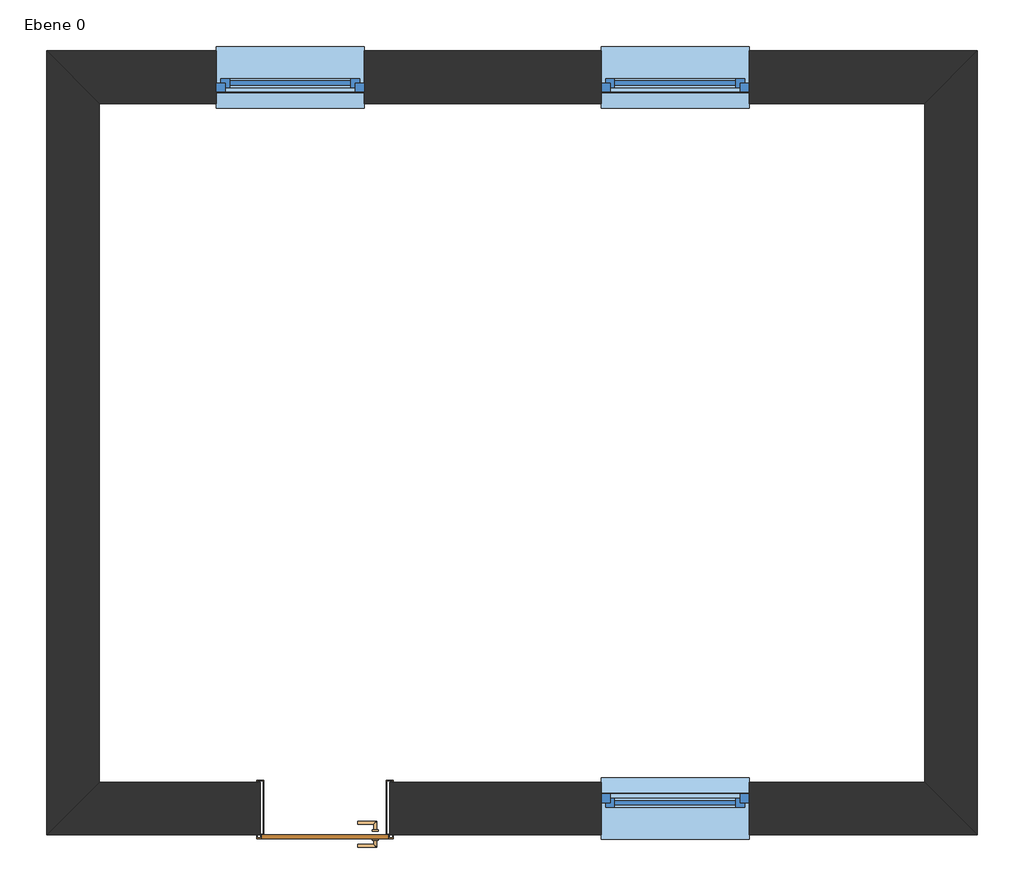
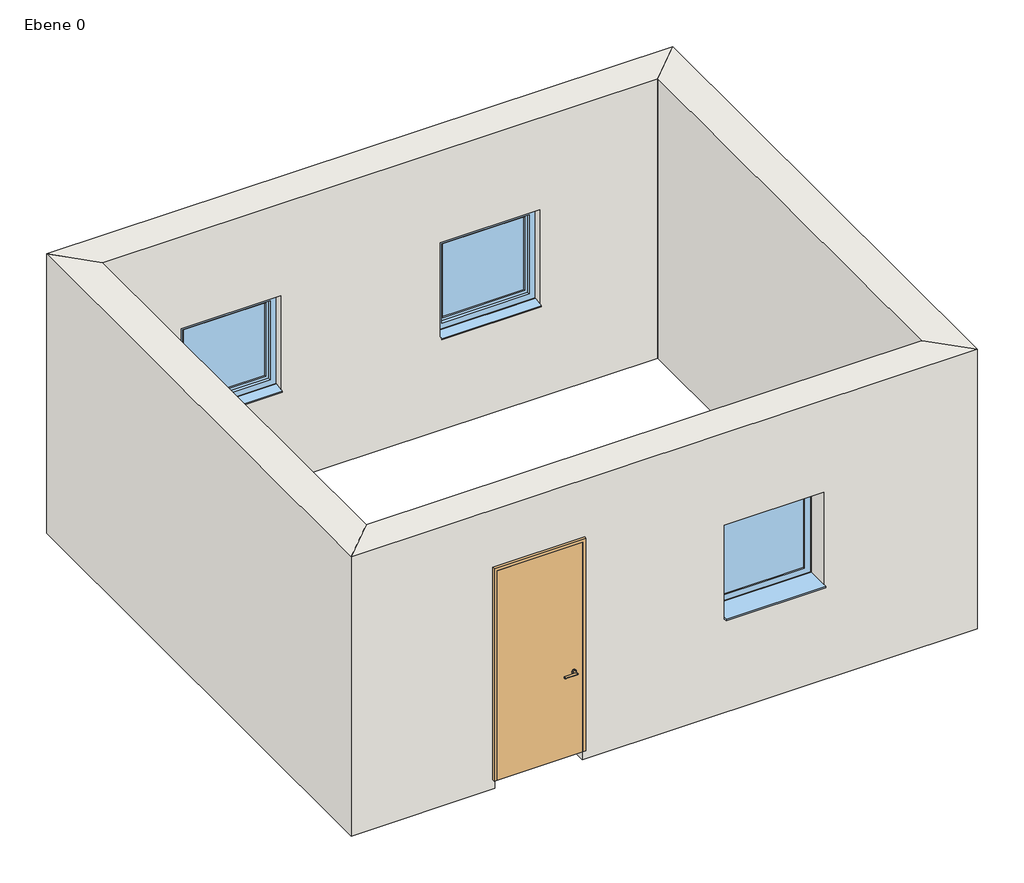
# One storey: 4 walls, 3 windows, 1 door.
"""IFC4 building model written with IfcOpenShell, lengths in millimetres."""

import ifcopenshell
import ifcopenshell.guid

model = None  # the IFC model being written
_history = None  # IfcOwnerHistory: only IFC2X3 demands one
_inside = {}  # id of a spatial element -> (the spatial element, [elements in it])
_under = {}  # id of a project, library or spatial element -> (it, [spatial elements below it])
_declared = {}  # id of a project -> (the project, [libraries it declares])
_typed = {}  # id of a type object -> (the type object, [elements of that type])
_made_of = {}  # id of a material, layer set ... -> (it, [elements and type objects made of it])


def new_model(schema):
    """Start an empty IFC model of exactly this schema.

    Asked for "IFC4X3", IfcOpenShell would pick the latest addendum, in which some entities
    have other attributes; the version numbers below select the first issue.
    IFC2X3 requires an IfcOwnerHistory on every rooted entity: one is made here for all.
    """
    global model, _history
    if schema == "IFC4X3":
        model = ifcopenshell.file(schema_version=(4, 3, 0, 0))
    else:
        model = ifcopenshell.file(schema=schema)
    _inside.clear()
    _under.clear()
    _declared.clear()
    _typed.clear()
    _made_of.clear()
    _history = None
    if model.schema == "IFC2X3":
        org = make("IfcOrganization", Name="unknown")
        user = make(
            "IfcPersonAndOrganization",
            ThePerson=make("IfcPerson", FamilyName="unknown"),
            TheOrganization=org,
        )
        app = make(
            "IfcApplication",
            ApplicationDeveloper=org,
            Version="unknown",
            ApplicationFullName="unknown",
            ApplicationIdentifier="unknown",
        )
        _history = make(
            "IfcOwnerHistory",
            OwningUser=user,
            OwningApplication=app,
            ChangeAction="ADDED",
            CreationDate=0,
        )
    return model


def make(cls, **values):
    """One entity of the class cls with the attributes given. An attribute that is None is left unset."""
    return model.create_entity(
        cls, **{name: value for name, value in values.items() if value is not None}
    )


def rooted(cls, **values):
    """An entity with a GlobalId (a new one), such as an element, a storey or a relation."""
    return make(cls, GlobalId=ifcopenshell.guid.new(), OwnerHistory=_history, **values)


def si_unit(unit_type, name, prefix=None):
    """IfcSIUnit, for example si_unit("LENGTHUNIT", "METRE", prefix="MILLI")."""
    return make("IfcSIUnit", UnitType=unit_type, Prefix=prefix, Name=name)


def assignment(units):
    """IfcUnitAssignment: the units of a project."""
    return None if units is None else make("IfcUnitAssignment", Units=units)


def point(xyz):
    """IfcCartesianPoint."""
    return None if xyz is None else make("IfcCartesianPoint", Coordinates=xyz)


def direction(xyz):
    """IfcDirection."""
    return None if xyz is None else make("IfcDirection", DirectionRatios=xyz)


def frame(location, z_axis=None, x_axis=None):
    """IfcAxis2Placement3D, a coordinate frame: its origin and axes. An axis left out is left unset."""
    return make(
        "IfcAxis2Placement3D",
        Location=point(location),
        Axis=direction(z_axis),
        RefDirection=direction(x_axis),
    )


def frame_2d(location, x_axis=None):
    """IfcAxis2Placement2D, a coordinate frame in the plane: its origin and x axis."""
    return make(
        "IfcAxis2Placement2D", Location=point(location), RefDirection=direction(x_axis)
    )


def origin():
    """The frame at (0, 0, 0) with its axes left unset."""
    return frame((0.0, 0.0, 0.0))


def origin_with_axes():
    """The frame at (0, 0, 0) with the z axis (0, 0, 1) and the x axis (1, 0, 0) written out."""
    return frame((0.0, 0.0, 0.0), z_axis=(0.0, 0.0, 1.0), x_axis=(1.0, 0.0, 0.0))


def place(relative_to, where):
    """IfcLocalPlacement: puts the frame where relative to a parent placement (None: the world)."""
    return make(
        "IfcLocalPlacement", PlacementRelTo=relative_to, RelativePlacement=where
    )


def context(
    kind, dimensions, precision=None, world=None, true_north=None, identifier=None
):
    """IfcGeometricRepresentationContext, for example the 3D "Model" context."""
    return make(
        "IfcGeometricRepresentationContext",
        ContextIdentifier=identifier,
        ContextType=kind,
        CoordinateSpaceDimension=dimensions,
        Precision=precision,
        WorldCoordinateSystem=world,
        TrueNorth=true_north,
    )


def project(units=None, contexts=None):
    """IfcProject with its units and contexts."""
    return rooted(
        "IfcProject",
        Name="project",
        RepresentationContexts=contexts,
        UnitsInContext=assignment(units),
    )


def spatial(cls, under=None, at=None, **own):
    """A site, building, storey or space (cls), placed at a placement, below another one or the project."""
    s = rooted(cls, ObjectPlacement=at, **own)
    if under is not None:
        _under.setdefault(under.id(), (under, []))[1].append(s)
    return s


def polyline(points):
    """IfcPolyline through the points."""
    return make("IfcPolyline", Points=[point(p) for p in points])


def circle_curve(where, radius):
    """IfcCircle in the frame where."""
    return make("IfcCircle", Position=where, Radius=radius)


def ellipse_curve(where, semi_axis1, semi_axis2):
    """IfcEllipse in the frame where."""
    return make(
        "IfcEllipse", Position=where, SemiAxis1=semi_axis1, SemiAxis2=semi_axis2
    )


def trimmed(basis, trim1, trim2, sense, master):
    """IfcTrimmedCurve: the piece of a basis curve between two trims."""
    return make(
        "IfcTrimmedCurve",
        BasisCurve=basis,
        Trim1=trim1,
        Trim2=trim2,
        SenseAgreement=sense,
        MasterRepresentation=master,
    )


def segment(curve, same_sense, transition):
    """IfcCompositeCurveSegment."""
    return make(
        "IfcCompositeCurveSegment",
        Transition=transition,
        SameSense=same_sense,
        ParentCurve=curve,
    )


def composite_curve(segments, self_intersect=None):
    """IfcCompositeCurve: segments joined end to end."""
    return make("IfcCompositeCurve", Segments=segments, SelfIntersect=self_intersect)


def outline(outer, holes=None, kind="AREA"):
    """IfcArbitraryClosedProfileDef: a profile drawn as a closed curve; with holes, ...WithVoids."""
    if holes is None:
        return make("IfcArbitraryClosedProfileDef", ProfileType=kind, OuterCurve=outer)
    return make(
        "IfcArbitraryProfileDefWithVoids",
        ProfileType=kind,
        OuterCurve=outer,
        InnerCurves=holes,
    )


def extrude(swept, where, along, depth):
    """IfcExtrudedAreaSolid: the profile swept, set in the frame where, extruded along a direction by depth."""
    return make(
        "IfcExtrudedAreaSolid",
        SweptArea=swept,
        Position=where,
        ExtrudedDirection=direction(along),
        Depth=depth,
    )


def faces_of(points, faces, orient=None, outer=None):
    """IfcFace entities. A face is a list of loops; a loop is a list of indices into points, from 0.

    orient and outer hold one flag for each loop. By default every Orientation is true, the
    first loop of a face is its IfcFaceOuterBound and the others are IfcFaceBound.
    """
    made = []
    for i, loops in enumerate(faces):
        bounds = []
        for j, loop in enumerate(loops):
            is_outer = j == 0 if outer is None else outer[i][j]
            bounds.append(
                make(
                    "IfcFaceOuterBound" if is_outer else "IfcFaceBound",
                    Bound=make("IfcPolyLoop", Polygon=[points[k] for k in loop]),
                    Orientation=True if orient is None else orient[i][j],
                )
            )
        made.append(make("IfcFace", Bounds=bounds))
    return made


def faceted_brep(points, faces, orient=None, outer=None, voids=None):
    """IfcFacetedBrep: a solid bounded by flat faces; with voids (closed shells), ...WithVoids."""
    shared = [point(p) for p in points]
    hull = make("IfcClosedShell", CfsFaces=faces_of(shared, faces, orient, outer))
    if voids is None:
        return make("IfcFacetedBrep", Outer=hull)
    return make(
        "IfcFacetedBrepWithVoids",
        Outer=hull,
        Voids=[
            make(cls, CfsFaces=faces_of(shared, fs, o, b)) for cls, fs, o, b in voids
        ],
    )


def shape(context_of_items, identifier, shape_type, items):
    """IfcShapeRepresentation: the items that make up one representation, for example the "Body"."""
    return make(
        "IfcShapeRepresentation",
        ContextOfItems=context_of_items,
        RepresentationIdentifier=identifier,
        RepresentationType=shape_type,
        Items=items,
    )


def source(mapping_origin, context_of_items, identifier, shape_type, items):
    """IfcRepresentationMap: a shape defined once, which mapped items show again and again."""
    return make(
        "IfcRepresentationMap",
        MappingOrigin=mapping_origin,
        MappedRepresentation=shape(context_of_items, identifier, shape_type, items),
    )


def transform(
    local_origin,
    x_axis=None,
    y_axis=None,
    z_axis=None,
    scale=None,
    scale2=None,
    scale3=None,
    uniform=True,
):
    """IfcCartesianTransformationOperator3D, or its non-uniform kind. x_axis, y_axis, z_axis: its Axis1, 2, 3."""
    if uniform:
        return make(
            "IfcCartesianTransformationOperator3D",
            Axis1=direction(x_axis),
            Axis2=direction(y_axis),
            LocalOrigin=point(local_origin),
            Scale=scale,
            Axis3=direction(z_axis),
        )
    return make(
        "IfcCartesianTransformationOperator3DnonUniform",
        Axis1=direction(x_axis),
        Axis2=direction(y_axis),
        LocalOrigin=point(local_origin),
        Scale=scale,
        Axis3=direction(z_axis),
        Scale2=scale2,
        Scale3=scale3,
    )


def mapped(mapping_source, mapping_target):
    """IfcMappedItem: shows the shape of a source again, moved by a transform."""
    return make(
        "IfcMappedItem", MappingSource=mapping_source, MappingTarget=mapping_target
    )


def made_of(thing, what):
    """Note that an element or type object is made of a material, layer set ...; save() writes the relation."""
    if what is not None:
        _made_of.setdefault(what.id(), (what, []))[1].append(thing)
    return thing


def element(
    cls,
    number,
    at=None,
    inside=None,
    cuts=None,
    type_object=None,
    material=None,
    context=None,
    identifier="Body",
    shape_type=None,
    held_by="IfcProductDefinitionShape",
    body=None,
    shapes=None,
    **own,
):
    """One element of the class cls, such as IfcWall. Its Tag is "e" and its number.

    at: its placement. inside: the storey or other place that contains it. cuts: it is an
    opening in that element (IfcRelVoidsElement). A single representation is given by context,
    identifier, shape_type and body (its items); several are given by shapes. held_by: the class
    of the entity that holds the representations. save() writes the other relations.
    """
    e = rooted(cls, Tag="e%d" % number, ObjectPlacement=at, **own)
    if body is not None:
        shapes = [shape(context, identifier, shape_type, body)]
    if shapes is not None:
        e.Representation = make(held_by, Representations=shapes)
    if inside is not None:
        _inside.setdefault(inside.id(), (inside, []))[1].append(e)
    if cuts is not None:
        rooted(
            "IfcRelVoidsElement", RelatingBuildingElement=cuts, RelatedOpeningElement=e
        )
    if type_object is not None:
        _typed.setdefault(type_object.id(), (type_object, []))[1].append(e)
    return made_of(e, material)


def aggregate(whole, parts):
    """IfcRelAggregates: a whole, such as a stair, and the parts it consists of."""
    return rooted("IfcRelAggregates", RelatingObject=whole, RelatedObjects=parts)


def save(model, path):
    """Write the relations noted so far, then the file.

    IfcRelAggregates (storeys below a building ...), IfcRelContainedInSpatialStructure (elements
    in a storey), IfcRelDefinesByType, IfcRelAssociatesMaterial and IfcRelDeclares: one each for
    every whole, place, type object, material and project.
    """
    for whole, parts in _under.values():
        aggregate(whole, parts)
    for where, things in _inside.values():
        rooted(
            "IfcRelContainedInSpatialStructure",
            RelatedElements=things,
            RelatingStructure=where,
        )
    for kind, things in _typed.values():
        rooted("IfcRelDefinesByType", RelatedObjects=things, RelatingType=kind)
    for what, things in _made_of.values():
        rooted("IfcRelAssociatesMaterial", RelatedObjects=things, RelatingMaterial=what)
    for by, libraries in _declared.values():
        rooted("IfcRelDeclares", RelatingContext=by, RelatedDefinitions=libraries)
    model.write(path)


def plane_surface(at):
    """IfcPlane: the flat surface through the origin of the frame at, square to its z axis."""
    return make("IfcPlane", Position=at)


def cylinder_surface(at, radius):
    """IfcCylindricalSurface: all points at the distance radius from the z axis of the frame at."""
    return make("IfcCylindricalSurface", Position=at, Radius=radius)


def advanced_brep(points, edges, surfaces, faces):
    """IfcAdvancedBrep: a solid bounded by faces that lie on surfaces and meet in shared edges.

    An edge is (start, end): straight between two places in points (the first is 0);
    or (start, end, curve); or (start, end, curve, False) where it runs against its curve.
    A face is (place in surfaces, loops), or (place, loops, False) where it looks against
    its surface's normal. A loop lists edges by number (the first is 1), with a minus sign
    where the edge is run from its end to its start. The first loop is the outer one.
    """
    corners = [point(p) for p in points]
    vertices = [make("IfcVertexPoint", VertexGeometry=c) for c in corners]
    made = []
    for start, end, *more in edges:
        made.append(
            make(
                "IfcEdgeCurve",
                EdgeStart=vertices[start],
                EdgeEnd=vertices[end],
                EdgeGeometry=more[0] if more else make("IfcPolyline", Points=[corners[start], corners[end]]),
                SameSense=more[1] if len(more) > 1 else True,
            )
        )
    hull = []
    for where, loops, *sense in faces:
        bounds = []
        for j, loop in enumerate(loops):
            ring = [make("IfcOrientedEdge", EdgeElement=made[abs(k) - 1], Orientation=k > 0) for k in loop]
            bounds.append(
                make(
                    "IfcFaceOuterBound" if j == 0 else "IfcFaceBound",
                    Bound=make("IfcEdgeLoop", EdgeList=ring),
                    Orientation=True,
                )
            )
        hull.append(make("IfcAdvancedFace", Bounds=bounds, FaceSurface=surfaces[where], SameSense=sense[0] if sense else True))
    return make("IfcAdvancedBrep", Outer=make("IfcClosedShell", CfsFaces=hull))


def door_88_5_x_2_26_80f06d6c(model_context):
    return source(origin(), model_context, "Body", "SolidModel", [
        advanced_brep(
        [(-352.5, 169.4346141, 1000.0), (-332.5, 169.4346141, 1000.0), (-352.5, 99.4346141, 1000.0), (-332.5, 119.4346141, 1000.0), (-222.5, 99.4346141, 1000.0), (-222.5, 119.4346141, 1000.0)],
        [
            (0, 1, circle_curve(frame((-342.5, 169.4346141, 1000.0), z_axis=(0.0, 1.0, 0.0), x_axis=(1.0, 0.0, 0.0)), 10.0)),
            (1, 0, circle_curve(frame((-342.5, 169.4346141, 1000.0), z_axis=(0.0, 1.0, 0.0), x_axis=(1.0, 0.0, 0.0)), 10.0)),
            (0, 2),
            (2, 3, ellipse_curve(frame((-342.5, 109.4346141, 1000.0), z_axis=(-0.7071067811865385, 0.7071067811865565, 0.0), x_axis=(0.7071067811865563, 0.7071067811865386, 0.0)), 14.1421356, 10.0)),
            (3, 1),
            (3, 2, ellipse_curve(frame((-342.5, 109.4346141, 1000.0), z_axis=(-0.7071067811865385, 0.7071067811865565, 0.0), x_axis=(0.7071067811865563, 0.7071067811865386, 0.0)), 14.1421356, 10.0)),
            (4, 5, circle_curve(frame((-222.5, 109.4346141, 1000.0), z_axis=(1.0, 0.0, 0.0), x_axis=(0.0, 1.0, 0.0)), 10.0)),
            (5, 4, circle_curve(frame((-222.5, 109.4346141, 1000.0), z_axis=(1.0, 0.0, 0.0), x_axis=(0.0, 1.0, 0.0)), 10.0)),
            (2, 4),
            (5, 3),
        ],
        [
            plane_surface(frame((-342.5, 169.4346141, -287.7526403), z_axis=(0.0, 1.0, 0.0), x_axis=(0.0, 0.0, 1.0))),
            cylinder_surface(frame((-342.5, 169.4346141, 1000.0), z_axis=(0.0, 1.0, 0.0), x_axis=(1.0, 0.0, 0.0)), 10.0),
            plane_surface(frame((-222.5, 109.4346141, -287.7526403), z_axis=(1.0, 0.0, 0.0), x_axis=(0.0, 0.0, 1.0))),
            cylinder_surface(frame((-342.5, 109.4346141, 1000.0), z_axis=(-1.0, 0.0, 0.0), x_axis=(0.0, 1.0, 0.0)), 10.0),
        ],
        [
            (0, [[1, 2]]),
            (1, [[-1, 3, 4, 5]]),
            (1, [[-2, -5, 6, -3]]),
            (2, [[7, 8]]),
            (3, [[-4, 9, -8, 10]]),
            (3, [[-6, -10, -7, -9]]),
        ],
    ),
        advanced_brep(
        [(-332.5, 229.4346141, 1000.0), (-352.5, 229.4346141, 1000.0), (-332.5, 259.4346141, 1000.0), (-352.5, 279.4346141, 1000.0), (-222.5, 259.4346141, 1000.0), (-222.5, 279.4346141, 1000.0)],
        [
            (0, 1, circle_curve(frame((-342.5, 229.4346141, 1000.0), z_axis=(0.0, -1.0, 0.0), x_axis=(-1.0, 0.0, 0.0)), 10.0)),
            (1, 0, circle_curve(frame((-342.5, 229.4346141, 1000.0), z_axis=(0.0, -1.0, 0.0), x_axis=(-1.0, 0.0, 0.0)), 10.0)),
            (0, 2),
            (2, 3, ellipse_curve(frame((-342.5, 269.4346141, 1000.0), z_axis=(-0.7071067811865475, -0.7071067811865475, 0.0), x_axis=(0.7071067811865474, -0.7071067811865476, 0.0)), 14.1421356, 10.0)),
            (3, 1),
            (3, 2, ellipse_curve(frame((-342.5, 269.4346141, 1000.0), z_axis=(-0.7071067811865475, -0.7071067811865475, 0.0), x_axis=(0.7071067811865474, -0.7071067811865476, 0.0)), 14.1421356, 10.0)),
            (4, 5, circle_curve(frame((-222.5, 269.4346141, 1000.0), z_axis=(1.0, 0.0, 0.0), x_axis=(0.0, 1.0, 0.0)), 10.0)),
            (5, 4, circle_curve(frame((-222.5, 269.4346141, 1000.0), z_axis=(1.0, 0.0, 0.0), x_axis=(0.0, 1.0, 0.0)), 10.0)),
            (2, 4),
            (5, 3),
        ],
        [
            plane_surface(frame((-342.5, 229.4346141, -287.7526403), z_axis=(0.0, -1.0, 0.0), x_axis=(0.0, 0.0, 1.0))),
            cylinder_surface(frame((-342.5, 229.4346141, 1000.0), z_axis=(0.0, -1.0, 0.0), x_axis=(-1.0, 0.0, 0.0)), 10.0),
            plane_surface(frame((-222.5, 269.4346141, -287.7526403), z_axis=(1.0, 0.0, 0.0), x_axis=(0.0, 0.0, 1.0))),
            cylinder_surface(frame((-342.5, 269.4346141, 1000.0), z_axis=(-1.0, 0.0, 0.0), x_axis=(0.0, 1.0, 0.0)), 10.0),
        ],
        [
            (0, [[1, 2]]),
            (1, [[-1, 3, 4, 5]]),
            (1, [[-2, -5, 6, -3]]),
            (2, [[7, 8]]),
            (3, [[-4, 9, -8, 10]]),
            (3, [[-6, -10, -7, -9]]),
        ],
    ),
        extrude(outline(composite_curve([segment(trimmed(circle_curve(frame_2d((1000.0, -342.5)), 20.0), [point((1000.0, -362.5))], [point((1000.0, -322.5))], False, "CARTESIAN"), True, "CONTINUOUS"), segment(trimmed(circle_curve(frame_2d((1000.0, -342.5)), 20.0), [point((1000.0, -322.5))], [point((1000.0, -362.5))], False, "CARTESIAN"), True, "CONTINUOUS")], self_intersect=False)), frame((0.0, 159.4346141, 0.0), z_axis=(0.0, 1.0, 0.0), x_axis=(0.0, 0.0, 1.0)), (0.0, 0.0, 1.0), 10.0),
        extrude(outline(composite_curve([segment(trimmed(circle_curve(frame_2d((1000.0, -342.5)), 20.0), [point((1000.0, -362.5))], [point((1000.0, -322.5))], False, "CARTESIAN"), True, "CONTINUOUS"), segment(trimmed(circle_curve(frame_2d((1000.0, -342.5)), 20.0), [point((1000.0, -322.5))], [point((1000.0, -362.5))], False, "CARTESIAN"), True, "CONTINUOUS")], self_intersect=False)), frame((0.0, 219.4346141, 0.0), z_axis=(0.0, 1.0, 0.0), x_axis=(0.0, 0.0, 1.0)), (0.0, 0.0, 1.0), 10.0),
        extrude(outline(polyline([(432.5, 194.4346141), (-432.5, 194.4346141), (-432.5, 219.4346141), (432.5, 219.4346141), (432.5, 194.4346141)])), frame((0.0, 0.0, 100.0), z_axis=(0.0, 0.0, 1.0), x_axis=(1.0, 0.0, 0.0)), (0.0, 0.0, 1.0), 2250.0),
        faceted_brep([(466.9603207, -180.5653859, 100.0), (417.5, -180.5653859, 100.0), (417.5, 194.4346141, 100.0), (432.5, 194.4346141, 100.0), (432.5, 219.4346141, 100.0), (466.9603207, 219.4346141, 100.0), (466.9603207, 194.4346141, 100.0), (461.9603207, 194.4346141, 100.0), (461.9603207, 214.4346141, 100.0), (437.5, 214.4346141, 100.0), (437.5, 189.4346141, 100.0), (422.5, 189.4346141, 100.0), (422.5, -175.5653859, 100.0), (461.9603207, -175.5653859, 100.0), (461.9603207, -165.5653859, 100.0), (466.9603207, -165.5653859, 100.0), (466.9603207, -180.5653859, 2384.4603207), (-466.9603207, -180.5653859, 2384.4603207), (-466.9603207, -180.5653859, 100.0), (-417.5, -180.5653859, 100.0), (-417.5, -180.5653859, 2335.0), (417.5, -180.5653859, 2335.0), (417.5, 194.4346141, 2335.0), (-417.5, 194.4346141, 2335.0), (-417.5, 194.4346141, 100.0), (-432.5, 194.4346141, 100.0), (-432.5, 194.4346141, 2350.0), (432.5, 194.4346141, 2350.0), (432.5, 219.4346141, 2350.0), (-432.5, 219.4346141, 2350.0), (-432.5, 219.4346141, 100.0), (-466.9603207, 219.4346141, 100.0), (-466.9603207, 219.4346141, 2384.4603207), (466.9603207, 219.4346141, 2384.4603207), (466.9603207, 194.4346141, 2384.4603207), (-466.9603207, 194.4346141, 2384.4603207), (-466.9603207, 194.4346141, 100.0), (-461.9603207, 194.4346141, 100.0), (-461.9603207, 194.4346141, 2379.4603207), (461.9603207, 194.4346141, 2379.4603207), (461.9603207, 214.4346141, 2379.4603207), (-461.9603207, 214.4346141, 2379.4603207), (-461.9603207, 214.4346141, 100.0), (-437.5, 214.4346141, 100.0), (-437.5, 214.4346141, 2355.0), (437.5, 214.4346141, 2355.0), (437.5, 189.4346141, 2355.0), (-437.5, 189.4346141, 2355.0), (-437.5, 189.4346141, 100.0), (-422.5, 189.4346141, 100.0), (-422.5, 189.4346141, 2340.0), (422.5, 189.4346141, 2340.0), (422.5, -175.5653859, 2340.0), (-422.5, -175.5653859, 2340.0), (-422.5, -175.5653859, 100.0), (-461.9603207, -175.5653859, 100.0), (-461.9603207, -175.5653859, 2379.4603207), (461.9603207, -175.5653859, 2379.4603207), (461.9603207, -165.5653859, 2379.4603207), (-461.9603207, -165.5653859, 2379.4603207), (-461.9603207, -165.5653859, 100.0), (-466.9603207, -165.5653859, 100.0), (-466.9603207, -165.5653859, 2384.4603207), (466.9603207, -165.5653859, 2384.4603207)], [[[0, 1, 2, 3, 4, 5, 6, 7, 8, 9, 10, 11, 12, 13, 14, 15]], [[1, 0, 16, 17, 18, 19, 20, 21]], [[2, 1, 21, 22]], [[3, 2, 22, 23, 24, 25, 26, 27]], [[4, 3, 27, 28]], [[5, 4, 28, 29, 30, 31, 32, 33]], [[6, 5, 33, 34]], [[7, 6, 34, 35, 36, 37, 38, 39]], [[8, 7, 39, 40]], [[9, 8, 40, 41, 42, 43, 44, 45]], [[10, 9, 45, 46]], [[11, 10, 46, 47, 48, 49, 50, 51]], [[12, 11, 51, 52]], [[13, 12, 52, 53, 54, 55, 56, 57]], [[14, 13, 57, 58]], [[15, 14, 58, 59, 60, 61, 62, 63]], [[0, 15, 63, 16]], [[17, 62, 61, 18]], [[18, 61, 60, 55, 54, 49, 48, 43, 42, 37, 36, 31, 30, 25, 24, 19]], [[23, 20, 19, 24]], [[29, 26, 25, 30]], [[35, 32, 31, 36]], [[41, 38, 37, 42]], [[47, 44, 43, 48]], [[53, 50, 49, 54]], [[59, 56, 55, 60]], [[22, 21, 20, 23]], [[28, 27, 26, 29]], [[34, 33, 32, 35]], [[40, 39, 38, 41]], [[46, 45, 44, 47]], [[52, 51, 50, 53]], [[58, 57, 56, 59]], [[16, 63, 62, 17]]]),
    ])


def fenster_1_flg_variabel_fenster_1_flg_variabel_3_8a378bad(model_context):
    return source(origin(), model_context, "Body", "SolidModel", [
        extrude(outline(polyline([(2010.0, 505.0), (2010.0, -505.0), (1000.0, -505.0), (1000.0, 505.0), (2010.0, 505.0)]), holes=[polyline([(1930.0, 445.0), (1080.0, 445.0), (1080.0, -445.0), (1930.0, -445.0), (1930.0, 445.0)])]), frame((0.0, 40.0, 0.0), z_axis=(0.0, 1.0, 0.0), x_axis=(0.0, 0.0, 1.0)), (0.0, 0.0, 1.0), 60.0),
        faceted_brep([(475.0, 40.0, 1960.0), (475.0, 10.0, 1960.0), (475.0, 10.0, 1050.0), (475.0, 40.0, 1050.0), (-475.0, 10.0, 1960.0), (-475.0, 10.0, 1050.0), (415.0, 10.0, 1110.0), (-415.0, 10.0, 1110.0), (-415.0, 10.0, 1900.0), (415.0, 10.0, 1900.0), (-475.0, 40.0, 1050.0), (-475.0, 40.0, 1960.0), (445.0, 40.0, 1930.0), (-445.0, 40.0, 1930.0), (-445.0, 40.0, 1080.0), (445.0, 40.0, 1080.0), (445.0, 70.0, 1930.0), (445.0, 70.0, 1080.0), (-445.0, 70.0, 1080.0), (-445.0, 70.0, 1930.0), (415.0, 70.0, 1900.0), (-415.0, 70.0, 1900.0), (-415.0, 70.0, 1110.0), (415.0, 70.0, 1110.0)], [[[0, 1, 2, 3]], [[1, 4, 5, 2], [6, 7, 8, 9]], [[3, 2, 5, 10]], [[3, 10, 11, 0], [12, 13, 14, 15]], [[16, 12, 15, 17]], [[17, 15, 14, 18]], [[17, 18, 19, 16], [20, 21, 22, 23]], [[9, 20, 23, 6]], [[6, 23, 22, 7]], [[10, 5, 4, 11]], [[18, 14, 13, 19]], [[7, 22, 21, 8]], [[11, 4, 1, 0]], [[19, 13, 12, 16]], [[8, 21, 20, 9]]]),
        extrude(outline(polyline([(-505.0, -210.0), (-505.0, 40.0), (505.0, 40.0), (505.0, -210.0), (-505.0, -210.0)])), frame((0.0, 0.0, 1005.0), z_axis=(0.0, 0.0, 1.0), x_axis=(1.0, 0.0, 0.0)), (0.0, 0.0, 1.0), 15.0),
        extrude(outline(polyline([(110.0221543, 1020.0), (210.0, 1000.0), (210.0, 990.0), (208.0, 990.0), (208.0, 998.3604634), (109.8240723, 1018.0), (100.0, 1018.0), (100.0, 1020.0), (110.0221543, 1020.0)])), frame((-505.0, 0.0, 0.0), z_axis=(1.0, 0.0, 0.0), x_axis=(0.0, 1.0, 0.0)), (0.0, 0.0, 1.0), 1010.0),
        extrude(outline(polyline([(415.0, 25.0), (-415.0, 25.0), (-415.0, 55.0), (415.0, 55.0), (415.0, 25.0)])), frame((0.0, 0.0, 1110.0), z_axis=(0.0, 0.0, 1.0), x_axis=(1.0, 0.0, 0.0)), (0.0, 0.0, 1.0), 790.0),
    ])


model = new_model("IFC4")

# Units and contexts
model_context = context("Model", 3, world=origin())
ifc_project = project(units=[si_unit("LENGTHUNIT", "METRE", prefix="MILLI")], contexts=[model_context])

# Site, building, storey
site = spatial("IfcSite", under=ifc_project)
building = spatial("IfcBuilding", under=site)
storey = spatial("IfcBuildingStorey", under=building, Name="Ebene 0", Elevation=0.0)

# Door
placement = place(None, origin())
door_88_5_x_2_26_shape = door_88_5_x_2_26_80f06d6c(model_context)
element("IfcDoor", 1, ObjectType="Drehflügel 1-flg - Stahlzarge : 88.5 x 2.26", at=placement, inside=storey, context=model_context, shape_type="MappedRepresentation", body=[
    mapped(door_88_5_x_2_26_shape, transform((-4461.0987005, 198.6603241, 0.0), x_axis=(-1.0, 0.0, 0.0), y_axis=(0.0, -1.0, 0.0), z_axis=(0.0, 0.0, 1.0))),
])

# Walls
element("IfcWall", 2, ObjectType="MW 24.0 WD 12.0", at=placement, inside=storey, context=model_context, shape_type="Brep", body=[
    faceted_brep([(-6003.5987005, 5004.2257101, 0.0), (-363.5987005, 5004.2257101, 0.0), (-363.5987005, 5004.2257101, 3000.0), (-6003.5987005, 5004.2257101, 3000.0), (-1563.5987005, 5004.2257101, 1000.0), (-2573.5987005, 5004.2257101, 1000.0), (-2573.5987005, 5004.2257101, 2010.0), (-1563.5987005, 5004.2257101, 2010.0), (-4193.5987005, 5004.2257101, 1000.0), (-5203.5987005, 5004.2257101, 1000.0), (-5203.5987005, 5004.2257101, 2010.0), (-4193.5987005, 5004.2257101, 2010.0), (-6363.5987005, 5364.2257101, 0.0), (-6363.5987005, 5364.2257101, 3000.0), (-3.5987005, 5364.2257101, 3000.0), (-3.5987005, 5364.2257101, 0.0), (-1563.5987005, 5364.2257101, 1000.0), (-1563.5987005, 5364.2257101, 2010.0), (-2573.5987005, 5364.2257101, 2010.0), (-2573.5987005, 5364.2257101, 1000.0), (-4193.5987005, 5364.2257101, 1000.0), (-4193.5987005, 5364.2257101, 2010.0), (-5203.5987005, 5364.2257101, 2010.0), (-5203.5987005, 5364.2257101, 1000.0)], [[[0, 1, 2, 3], [4, 5, 6, 7], [8, 9, 10, 11]], [[12, 13, 14, 15], [16, 17, 18, 19], [20, 21, 22, 23]], [[1, 0, 12, 15]], [[3, 2, 14, 13]], [[17, 16, 4, 7]], [[18, 17, 7, 6]], [[19, 18, 6, 5]], [[16, 19, 5, 4]], [[21, 20, 8, 11]], [[22, 21, 11, 10]], [[23, 22, 10, 9]], [[20, 23, 9, 8]], [[0, 3, 13, 12]], [[2, 1, 15, 14]]]),
])
element("IfcWall", 3, ObjectType="MW 24.0 WD 12.0", at=placement, inside=storey, context=model_context, shape_type="SweptSolid", body=[
    extrude(outline(polyline([(-363.5987005, 364.2257101), (-363.5987005, 5004.2257101), (-3.5987005, 5364.2257101), (-3.5987005, 4.2257101), (-363.5987005, 364.2257101)])), origin_with_axes(), (0.0, 0.0, 1.0), 3000.0),
])
element("IfcWall", 4, ObjectType="MW 24.0 WD 12.0", at=placement, inside=storey, context=model_context, shape_type="Brep", body=[
    faceted_brep([(-6003.5987005, 364.2257101, 3000.0), (-363.5987005, 364.2257101, 3000.0), (-363.5987005, 364.2257101, 0.0), (-4018.5987005, 364.2257101, 0.0), (-4018.5987005, 364.2257101, 2360.0), (-4903.5987005, 364.2257101, 2360.0), (-4903.5987005, 364.2257101, 0.0), (-6003.5987005, 364.2257101, 0.0), (-2573.5987005, 364.2257101, 1000.0), (-1563.5987005, 364.2257101, 1000.0), (-1563.5987005, 364.2257101, 2010.0), (-2573.5987005, 364.2257101, 2010.0), (-3.5987005, 4.2257101, 3000.0), (-6363.5987005, 4.2257101, 3000.0), (-6363.5987005, 4.2257101, 0.0), (-4903.5987005, 4.2257101, 0.0), (-4903.5987005, 4.2257101, 2360.0), (-4018.5987005, 4.2257101, 2360.0), (-4018.5987005, 4.2257101, 0.0), (-3.5987005, 4.2257101, 0.0), (-2573.5987005, 4.2257101, 1000.0), (-2573.5987005, 4.2257101, 2010.0), (-1563.5987005, 4.2257101, 2010.0), (-1563.5987005, 4.2257101, 1000.0)], [[[0, 1, 2, 3, 4, 5, 6, 7], [8, 9, 10, 11]], [[12, 13, 14, 15, 16, 17, 18, 19], [20, 21, 22, 23]], [[2, 19, 18, 3]], [[14, 7, 6, 15]], [[1, 0, 13, 12]], [[5, 16, 15, 6]], [[16, 5, 4, 17]], [[17, 4, 3, 18]], [[21, 20, 8, 11]], [[22, 21, 11, 10]], [[23, 22, 10, 9]], [[20, 23, 9, 8]], [[2, 1, 12, 19]], [[0, 7, 14, 13]]]),
])
element("IfcWall", 5, ObjectType="MW 24.0 WD 12.0", at=placement, inside=storey, context=model_context, shape_type="SweptSolid", body=[
    extrude(outline(polyline([(-6003.5987005, 5004.2257101), (-6003.5987005, 364.2257101), (-6363.5987005, 4.2257101), (-6363.5987005, 5364.2257101), (-6003.5987005, 5004.2257101)])), origin_with_axes(), (0.0, 0.0, 1.0), 3000.0),
])

# Windows
fenster_1_flg_variabel_fenster_1_flg_variabel_3_shape = fenster_1_flg_variabel_fenster_1_flg_variabel_3_8a378bad(model_context)
element("IfcWindow", 6, ObjectType="Fenster 1-flg - Variabel : Fenster 1-flg - Variabel 3", at=placement, inside=storey, context=model_context, shape_type="MappedRepresentation", body=[
    mapped(fenster_1_flg_variabel_fenster_1_flg_variabel_3_shape, transform((-2068.5987005, 184.2257101, 0.0), x_axis=(1.0, 0.0, 0.0), y_axis=(0.0, 1.0, 0.0), z_axis=(0.0, 0.0, 1.0))),
])
element("IfcWindow", 7, ObjectType="Fenster 1-flg - Variabel : Fenster 1-flg - Variabel 3", at=placement, inside=storey, context=model_context, shape_type="MappedRepresentation", body=[
    mapped(fenster_1_flg_variabel_fenster_1_flg_variabel_3_shape, transform((-2068.5987005, 5184.2257101, 0.0), x_axis=(-1.0, 0.0, 0.0), y_axis=(0.0, -1.0, 0.0), z_axis=(0.0, 0.0, 1.0))),
])
element("IfcWindow", 8, ObjectType="Fenster 1-flg - Variabel : Fenster 1-flg - Variabel 3", at=placement, inside=storey, context=model_context, shape_type="MappedRepresentation", body=[
    mapped(fenster_1_flg_variabel_fenster_1_flg_variabel_3_shape, transform((-4698.5987005, 5184.2257101, 0.0), x_axis=(-1.0, 0.0, 0.0), y_axis=(0.0, -1.0, 0.0), z_axis=(0.0, 0.0, 1.0))),
])

save(model, "model.ifc")

# Revit data of these elements
# Project information
#   Projektausgabedatum = "Projekt Datum"
#   Projektstatus = "Projektstatus"
#   Auftraggeber = "Walter Beispiel"
#   Projektadresse = "Zufallweg 2"
#   Projektname = "Projektname"
#   Projektnummer = "Projektnummer"
#   Verfasser Firma 1 = "Firma 1"
#   Verfasser Firma 2 = "Firma 2"
#   Verfasser PLZ Ort = "PLZ Ort"
#   Verfasser Strasse = "Strasse"
#   Verfasser Telefon = "Telefon"
#   Verfasser Telefax = "Telefax"
#   Verfasser eMail = "E-Mail"
# Type "Drehflügel 1-flg - Stahlzarge : 88.5 x 2.26"
#   Construction Type Id = "MDOOR"
#   Type Mark = "20"
#   Operation = "SingleSwingRight"
#   Keynote = "16.03"
#   Analytic Construction = "Metall"
#   Thermal Resistance (R) = 0.270117 (m²·K)/W
#   Heat Transfer Coefficient (U) = 3.7021 W/(m²·K)
#   Rough Width = 0.885 m
#   Rough Height [instance default] = 2.360 m
#   Höhe Türgriff [instance default] = 0.900 m
#   Height = 2.260 m
#   Fußbodenaufbau [instance default] = 0.100 m
#   Width = 0.885 m
#   Define Thermal Properties by = 1
#   Sichtbarkeit Sturzlinien [instance default] = yes
#   Türgriff auswählen [instance default] = element 221079
#   Türgriff [instance default] = none
#   Türflügel [instance default] = none
#   Rahmen/Pfosten [instance default] = Metall - Lackiert - Grau
#   Visual Light Transmittance = 0
#   Solar Heat Gain Coefficient = 0
#   Function = (empty or 0)
#   Wall Closure = (empty or 0)
# Type "MW 24.0 WD 12.0"
#   Type Comments = "Mehrschaliges Mauerwerk"
#   Description = "Mauerwerk 24.0 cm, Wärmedämmung 12.0 cm"
#   Layers, outside or top first: 0.120 m "Wärmedämmung - hart" (function 3); 0.240 m "Mauerwerk - Ziegel, verputzt" (function 1)
# Type "Fenster 1-flg - Variabel : Fenster 1-flg - Variabel 3"
#   Type Mark = "52"
#   Operation = "SinglePanel"
#   Construction Type Id = "GSP4R"
#   Keynote = "16.05.01"
#   Analytic Construction = "1/8 Zoll Pilkington-Verglasung einfach"
#   Cost = 78.2
#   Visual Light Transmittance = 0.9
#   Höhe oberer  Rahmen = 0.080 m
#   Solar Heat Gain Coefficient = 0.86
#   Tiefe Flügel = 0.060 m
#   Rough Width [instance default] = 1.010 m
#   Rough Height [instance default] = 1.010 m
#   Rahmenhöhe unten = 0.080 m
#   Heat Transfer Coefficient (U) = 6.7069 W/(m²·K)
#   Rahmentiefe = 0.060 m
#   Rahmenbreite = 0.060 m
#   Height [instance default] = 1.010 m
#   Flügelbreite = 0.060 m
#   Einbautiefe (von außen) [instance default] = 0.080 m
#   Width [instance default] = 1.010 m
#   Define Thermal Properties by = 1
#   Öffnungsrichtung oben [instance default] = yes
#   Öffnungsrichtung in Draufsicht anzeigen [instance default] = no
#   Klappflügel [instance default] = no
#   Drehflügel 1 [instance default] = yes
#   Fensterflügel [instance default] = none
#   Innere Fensterbank [instance default] = none
#   Glas [instance default] = none
#   Bild [instance default] = none
#   Äußere Fensterbank [instance default] = none
#   Wall Closure = (empty or 0)
# Element 1 (IfcDoor, "Drehflügel 1-flg - Stahlzarge : 88.5 x 2.26")
#   Rough Height = 2.360 m
#   Höhe Türgriff = 0.900 m
#   Fußbodenaufbau = 0.100 m
#   Sichtbarkeit Sturzlinien = yes
#   Türgriff auswählen = element 221079
#   Türgriff = none
#   Türflügel = none
#   Rahmen/Pfosten = Metall - Lackiert - Grau
#   Phase Created = Phase 1
#   Materials on its faces: "Metall - Lackiert - Grau", "Metall - Chrom", "Holz - Birke"
# Elements 2, 3, 4, 5 (IfcWall, "MW 24.0 WD 12.0")
#   Comments = ""
#   Top Offset = 0.000 m
#   Base Offset = 0.000 m
#   Unconnected Height = 3.000 m
#   wall height = 3.000 m
#   Phase Created = Phase 1
#   Base Constraint = Ebene 0
#   Materials on its faces: "Vorgabe - Wand", "Mauerwerk - Ziegel, verputzt", "Wärmedämmung - hart"
# Element 6 (IfcWindow, "Fenster 1-flg - Variabel : Fenster 1-flg - Variabel 3")
#   Mark = "1"
#   Rough Height = 1.010 m
#   Rough Width = 1.010 m
#   Height = 1.010 m
#   Einbautiefe (von außen) = 0.080 m
#   Width = 1.010 m
#   Öffnungsrichtung oben = yes
#   Öffnungsrichtung in Draufsicht anzeigen = no
#   Klappflügel = no
#   Drehflügel 1 = yes
#   Äußere Fensterbank = none
#   Innere Fensterbank = none
#   Glas = none
#   Fensterflügel = none
#   Bild = none
#   Phase Created = Phase 1
#   Materials on its faces: "Kunststoff - Weiß", "Holz - Birke", "Glas"
# Element 7 (IfcWindow, "Fenster 1-flg - Variabel : Fenster 1-flg - Variabel 3")
#   Mark = "6"
#   Rough Height = 1.010 m
#   Rough Width = 1.010 m
#   Height = 1.010 m
#   Einbautiefe (von außen) = 0.080 m
#   Width = 1.010 m
#   Öffnungsrichtung oben = yes
#   Öffnungsrichtung in Draufsicht anzeigen = no
#   Klappflügel = no
#   Drehflügel 1 = yes
#   Äußere Fensterbank = none
#   Innere Fensterbank = none
#   Glas = none
#   Fensterflügel = none
#   Bild = none
#   Phase Created = Phase 1
#   Materials on its faces: "Kunststoff - Weiß", "Holz - Birke", "Glas"
# Element 8 (IfcWindow, "Fenster 1-flg - Variabel : Fenster 1-flg - Variabel 3")
#   Mark = "7"
#   Rough Height = 1.010 m
#   Rough Width = 1.010 m
#   Height = 1.010 m
#   Einbautiefe (von außen) = 0.080 m
#   Width = 1.010 m
#   Öffnungsrichtung oben = yes
#   Öffnungsrichtung in Draufsicht anzeigen = no
#   Klappflügel = no
#   Drehflügel 1 = yes
#   Äußere Fensterbank = none
#   Innere Fensterbank = none
#   Glas = none
#   Fensterflügel = none
#   Bild = none
#   Phase Created = Phase 1
#   Materials on its faces: "Kunststoff - Weiß", "Holz - Birke", "Glas"
# Materials
#   "Metall - Lackiert - Grau": class "Farbe 1", colour RGB 98 98 98, transparency 0, Cost = 0
#   "Wärmedämmung - hart": class "Stuck", colour RGB 255 255 255, transparency 0, Description = "Äußere Oberfläche", Cost = 0
#   "Mauerwerk - Ziegel, verputzt": class "Stuck", colour RGB 247 247 247, transparency 0, Cost = 0
#   "Metall - Chrom": class "Metall", colour RGB 247 247 247, transparency 0, Cost = 0
#   "Holz - Birke": class "Holz", colour RGB 213 164 103, transparency 0, Cost = 0
#   "Vorgabe - Wand": class "Stuck", colour RGB 128 128 128, transparency 0, Description = "Äußere Oberfläche", Cost = 0
#   "Kunststoff - Weiß": class "Kunststoff", colour RGB 249 249 249, transparency 0, Cost = 0
#   "Glas": class "Glas", colour RGB 0 0 255, transparency 0.75, Comments = "Render-Darstellung nicht aktualisiert ", Cost = 0
